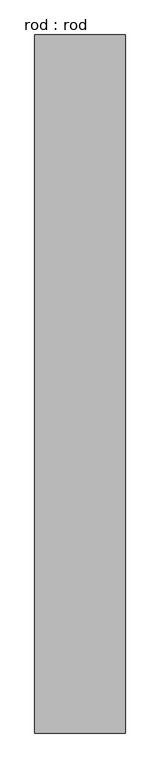
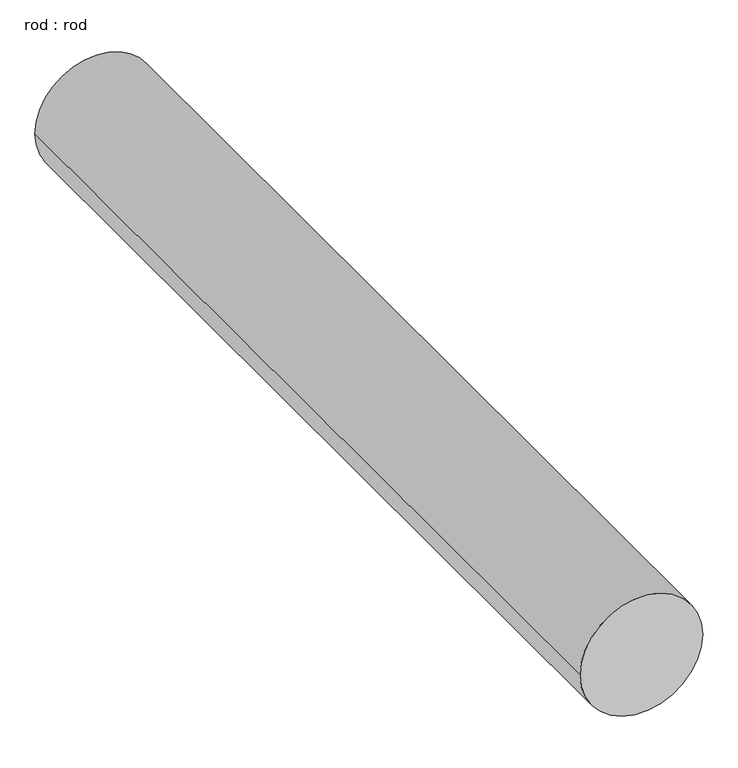
"""IFC4 building model written with IfcOpenShell, lengths in millimetres: proxy geometry, rod : rod."""

from ifc_helpers import new_model, si_unit, point, frame, frame_2d, origin, place, context, project, spatial, circle_curve, trimmed, segment, composite_curve, outline, extrude, source, transform, mapped, element, save


def rod_rod_fff75ba7(model_context):
    return source(origin(), model_context, "Body", "SweptSolid", [
        extrude(outline(composite_curve([segment(trimmed(circle_curve(frame_2d((0.0108462, 0.0)), 200.0), [point((0.0108462, 200.0))], [point((0.0108462, -200.0))], False, "CARTESIAN"), True, "CONTINUOUS"), segment(trimmed(circle_curve(frame_2d((0.0108462, 0.0)), 200.0), [point((0.0108462, -200.0))], [point((0.0108462, 200.0))], False, "CARTESIAN"), True, "CONTINUOUS")], self_intersect=False)), frame((0.0, 2552.7286153, 0.0), z_axis=(0.0, 1.0, 0.0), x_axis=(0.0, 0.0, 1.0)), (0.0, 0.0, 1.0), 3080.0),
    ])


if __name__ == "__main__":
    model = new_model("IFC4")
    model_context = context("Model", 3, world=origin())
    ifc_project = project(units=[si_unit("LENGTHUNIT", "METRE", prefix="MILLI")], contexts=[model_context])
    site = spatial("IfcSite", under=ifc_project)
    building = spatial("IfcBuilding", under=site)
    placement = place(None, origin())
    rod_rod_shape = rod_rod_fff75ba7(model_context)
    element("IfcBuildingElementProxy", 1, Name="rod : rod", ObjectType="rod : rod", at=placement, inside=building, context=model_context, shape_type="MappedRepresentation", body=[
        mapped(rod_rod_shape, transform((0.0, 0.0, 0.0), x_axis=(1.0, 0.0, 0.0), y_axis=(0.0, 1.0, 0.0), z_axis=(0.0, 0.0, 1.0))),
    ])
    save(model, "model.ifc")

# Revit data of these elements
# Type "rod : rod"
#   Default Elevation = 0
